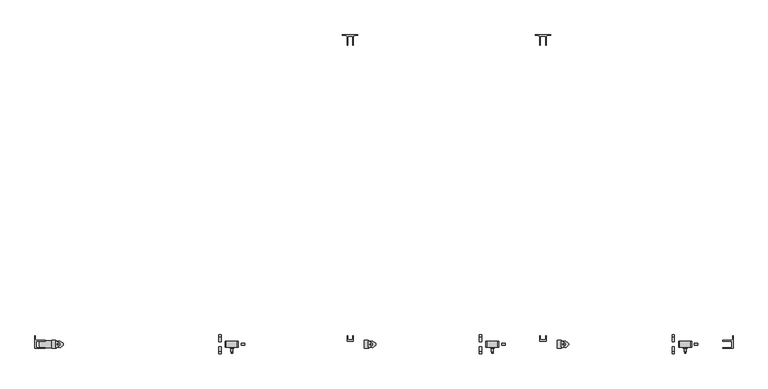
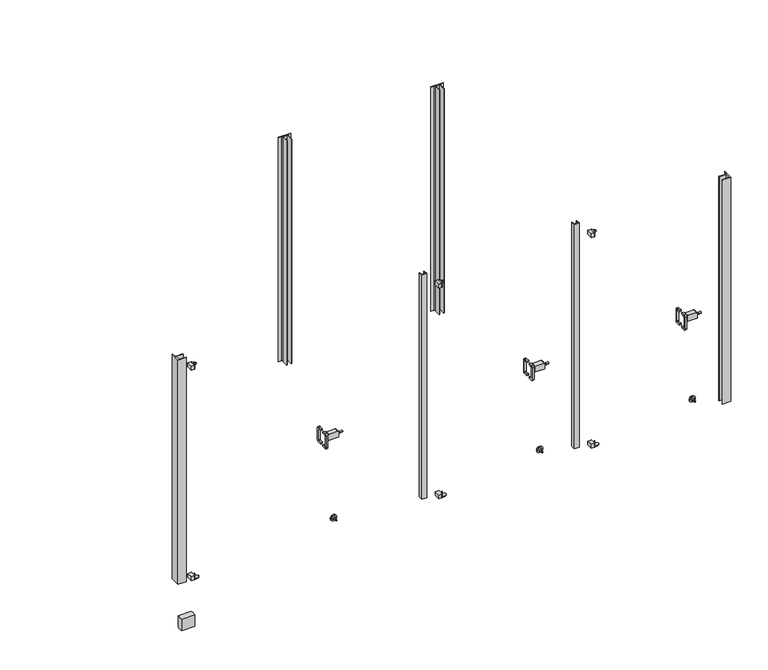
"""IFC4 building model written with IfcOpenShell, lengths in millimetres: proxy geometry, Partition-Floor_Braced-Bradley_Corp-St_Stl-ADA-N_Stalls : ADA (optional) + n Standard Stalls."""

from ifc_helpers import new_model, si_unit, point, frame, frame_2d, origin, origin_with_axes, place, context, project, spatial, polyline, circle_curve, ellipse_curve, trimmed, segment, composite_curve, outline, extrude, source, transform, mapped, element, save
from ifc_brep_helpers import plane_surface, cylinder_surface, revolved_surface, advanced_brep


def specialty_equipment_1cc22914(model_context):
    return source(origin(), model_context, "Body", "SolidModel", [
        extrude(outline(composite_curve([segment(trimmed(circle_curve(frame_2d((-1469.3891724, 977.9)), 10.16), [point((-1469.3891724, 988.06))], [point((-1459.2291724, 977.9))], False, "CARTESIAN"), True, "CONTINUOUS"), segment(polyline([(-1459.2291724, 977.9), (-1459.2291724, 901.7)]), True, "CONTINUOUS"), segment(trimmed(circle_curve(frame_2d((-1469.3891724, 901.7)), 10.16), [point((-1459.2291724, 901.7))], [point((-1469.3891724, 891.54))], False, "CARTESIAN"), True, "CONTINUOUS"), segment(polyline([(-1469.3891724, 891.54), (-1492.2491724, 891.54), (-1492.2491724, 901.7), (-1469.3891724, 901.7)]), True, "CONTINUOUS"), segment(trimmed(circle_curve(frame_2d((-1469.3891724, 904.24)), 2.54), [point((-1469.3891724, 901.7))], [point((-1466.8491724, 904.24))], True, "CARTESIAN"), True, "CONTINUOUS"), segment(polyline([(-1466.8491724, 904.24), (-1466.8491724, 975.36)]), True, "CONTINUOUS"), segment(trimmed(circle_curve(frame_2d((-1469.3891724, 975.36)), 2.54), [point((-1466.8491724, 975.36))], [point((-1469.3891724, 977.9))], True, "CARTESIAN"), True, "CONTINUOUS"), segment(polyline([(-1469.3891724, 977.9), (-1492.2491724, 977.9), (-1492.2491724, 988.06), (-1469.3891724, 988.06)]), True, "CONTINUOUS")], self_intersect=False)), frame((1086.5228738, 0.0, 0.0), z_axis=(1.0, 0.0, 0.0), x_axis=(0.0, 1.0, 0.0)), (0.0, 0.0, 1.0), 11.4113578),
        extrude(outline(composite_curve([segment(polyline([(-1540.51, 988.06), (-1517.65, 988.06), (-1517.65, 977.9), (-1540.51, 977.9)]), True, "CONTINUOUS"), segment(trimmed(circle_curve(frame_2d((-1540.51, 975.36)), 2.54), [point((-1540.51, 977.9))], [point((-1543.05, 975.36))], True, "CARTESIAN"), True, "CONTINUOUS"), segment(polyline([(-1543.05, 975.36), (-1543.05, 904.24)]), True, "CONTINUOUS"), segment(trimmed(circle_curve(frame_2d((-1540.51, 904.24)), 2.54), [point((-1543.05, 904.24))], [point((-1540.51, 901.7))], True, "CARTESIAN"), True, "CONTINUOUS"), segment(polyline([(-1540.51, 901.7), (-1517.65, 901.7), (-1517.65, 891.54), (-1540.51, 891.54)]), True, "CONTINUOUS"), segment(trimmed(circle_curve(frame_2d((-1540.51, 901.7)), 10.16), [point((-1540.51, 891.54))], [point((-1550.67, 901.7))], False, "CARTESIAN"), True, "CONTINUOUS"), segment(polyline([(-1550.67, 901.7), (-1550.67, 977.9)]), True, "CONTINUOUS"), segment(trimmed(circle_curve(frame_2d((-1540.51, 977.9)), 10.16), [point((-1550.67, 977.9))], [point((-1540.51, 988.06))], False, "CARTESIAN"), True, "CONTINUOUS")], self_intersect=False)), frame((1086.5228738, 0.0, 0.0), z_axis=(1.0, 0.0, 0.0), x_axis=(0.0, 1.0, 0.0)), (0.0, 0.0, 1.0), 11.4113578),
        extrude(outline(composite_curve([segment(trimmed(circle_curve(frame_2d((406.4, 1150.9250547)), 3.4532283), [point((402.9467717, 1150.9250547))], [point((409.8532283, 1150.9250547))], False, "CARTESIAN"), True, "CONTINUOUS"), segment(trimmed(circle_curve(frame_2d((406.4, 1150.9250547)), 3.4532283), [point((409.8532283, 1150.9250547))], [point((402.9467717, 1150.9250547))], False, "CARTESIAN"), True, "CONTINUOUS")], self_intersect=False)), frame((0.0, -1548.13, 0.0), z_axis=(0.0, 1.0, 0.0), x_axis=(0.0, 0.0, 1.0)), (0.0, 0.0, 1.0), 7.62),
        advanced_brep(
        [(1150.9250547, -1517.65, 406.4), (1131.8750547, -1517.65, 406.4), (1169.9750547, -1517.65, 406.4), (1156.0050547, -1540.51, 406.4), (1145.8450547, -1540.51, 406.4), (1150.9250547, -1540.51, 406.4), (1156.0050547, -1525.27, 406.4), (1145.8450547, -1525.27, 406.4), (1161.0850547, -1520.19, 406.4), (1140.7650547, -1520.19, 406.4), (1169.9750547, -1520.19, 406.4), (1131.8750547, -1520.19, 406.4)],
        [
            (0, 1),
            (1, 2, circle_curve(frame((1150.9250547, -1517.65, 406.4), z_axis=(0.0, 1.0, 0.0), x_axis=(-1.0, 0.0, 0.0)), 19.05)),
            (2, 0),
            (2, 1, circle_curve(frame((1150.9250547, -1517.65, 406.4), z_axis=(0.0, 1.0, 0.0), x_axis=(-1.0, 0.0, 0.0)), 19.05)),
            (3, 4, circle_curve(frame((1150.9250547, -1540.51, 406.4), z_axis=(0.0, -1.0, 0.0), x_axis=(-1.0, 0.0, 0.0)), 5.08)),
            (4, 5),
            (5, 3),
            (4, 3, circle_curve(frame((1150.9250547, -1540.51, 406.4), z_axis=(0.0, -1.0, 0.0), x_axis=(-1.0, 0.0, 0.0)), 5.08)),
            (6, 7, circle_curve(frame((1150.9250547, -1525.27, 406.4), z_axis=(0.0, -1.0, 0.0), x_axis=(-1.0, 0.0, 0.0)), 5.08)),
            (7, 4),
            (3, 6),
            (7, 6, circle_curve(frame((1150.9250547, -1525.27, 406.4), z_axis=(0.0, -1.0, 0.0), x_axis=(-1.0, 0.0, 0.0)), 5.08)),
            (8, 9, circle_curve(frame((1150.9250547, -1520.19, 406.4), z_axis=(0.0, -1.0, 0.0), x_axis=(-1.0, 0.0, 0.0)), 10.16)),
            (9, 7, circle_curve(frame((1145.8450547, -1520.19, 406.4), z_axis=(0.0, 0.0, 1.0), x_axis=(0.0, -1.0, 0.0)), 5.08)),
            (6, 8, circle_curve(frame((1156.0050547, -1520.19, 406.4), z_axis=(0.0, 0.0, 1.0), x_axis=(0.0, -1.0, 0.0)), 5.08)),
            (9, 8, circle_curve(frame((1150.9250547, -1520.19, 406.4), z_axis=(0.0, -1.0, 0.0), x_axis=(-1.0, 0.0, 0.0)), 10.16)),
            (10, 11, circle_curve(frame((1150.9250547, -1520.19, 406.4), z_axis=(0.0, -1.0, 0.0), x_axis=(-1.0, 0.0, 0.0)), 19.05)),
            (11, 9),
            (8, 10),
            (11, 10, circle_curve(frame((1150.9250547, -1520.19, 406.4), z_axis=(0.0, -1.0, 0.0), x_axis=(-1.0, 0.0, 0.0)), 19.05)),
            (1, 11),
            (10, 2),
        ],
        [
            plane_surface(frame((1150.9250547, -1517.65, 406.4), z_axis=(0.0, 1.0, 0.0), x_axis=(-1.0, 0.0, 0.0))),
            plane_surface(frame((1150.9250547, -1540.51, 406.4), z_axis=(0.0, -1.0, 0.0), x_axis=(-1.0, 0.0, 0.0))),
            cylinder_surface(frame((1150.9250547, -1561.6297247, 406.4), z_axis=(0.0, 1.0, 0.0), x_axis=(-1.0, 0.0, 0.0)), 5.08),
            revolved_surface(trimmed(ellipse_curve(frame((1145.8450547, -1520.19, 406.4), z_axis=(0.0, 0.0, -1.0), x_axis=(0.0, -1.0, 0.0)), 5.08, 5.08), [point((1145.8450547, -1525.27, 406.4))], [point((1140.7650547, -1520.19, 406.4))], True, "CARTESIAN"), (1150.9250547, -1561.6297247, 406.4), (0.0, 1.0, 0.0)),
            plane_surface(frame((1150.9250547, -1520.19, 406.4), z_axis=(0.0, -1.0, 0.0), x_axis=(-1.0, 0.0, 0.0))),
            cylinder_surface(frame((1150.9250547, -1561.6297247, 406.4), z_axis=(0.0, 1.0, 0.0), x_axis=(-1.0, 0.0, 0.0)), 19.05),
        ],
        [
            (0, [[1, 2, 3]]),
            (0, [[-3, 4, -1]]),
            (1, [[5, 6, 7]]),
            (1, [[8, -7, -6]]),
            (2, [[9, 10, -5, 11]]),
            (2, [[12, -11, -8, -10]]),
            (3, [[13, 14, -9, 15]]),
            (3, [[16, -15, -12, -14]]),
            (4, [[17, 18, -13, 19]]),
            (4, [[20, -19, -16, -18]]),
            (5, [[-2, 21, -17, 22]]),
            (5, [[-4, -22, -20, -21]]),
        ],
    ),
        advanced_brep(
        [(1195.3750547, -1499.87, 939.8), (1195.3750547, -1510.03, 939.8), (1212.8502547, -1510.03, 939.8), (1212.8502547, -1499.87, 939.8), (1195.3750547, -1504.95, 939.8), (1212.8502547, -1504.95, 939.8)],
        [
            (0, 1, circle_curve(frame((1195.3750547, -1504.95, 939.8), z_axis=(1.0, 0.0, 0.0), x_axis=(0.0, -1.0, 0.0)), 5.08)),
            (1, 2),
            (2, 3, circle_curve(frame((1212.8502547, -1504.95, 939.8), z_axis=(-1.0, 0.0, 0.0), x_axis=(0.0, -1.0, 0.0)), 5.08)),
            (3, 0),
            (1, 0, circle_curve(frame((1195.3750547, -1504.95, 939.8), z_axis=(1.0, 0.0, 0.0), x_axis=(0.0, -1.0, 0.0)), 5.08)),
            (3, 2, circle_curve(frame((1212.8502547, -1504.95, 939.8), z_axis=(-1.0, 0.0, 0.0), x_axis=(0.0, -1.0, 0.0)), 5.08)),
            (4, 1),
            (0, 4),
            (2, 5),
            (5, 3),
        ],
        [
            cylinder_surface(frame((1212.8502547, -1504.95, 939.8), z_axis=(-1.0, 0.0, 0.0), x_axis=(0.0, -1.0, 0.0)), 5.08),
            plane_surface(frame((1195.3750547, -1504.95, 939.8), z_axis=(-1.0, 0.0, 0.0), x_axis=(0.0, -1.0, 0.0))),
            plane_surface(frame((1212.8502547, -1504.95, 939.8), z_axis=(1.0, 0.0, 0.0), x_axis=(0.0, -1.0, 0.0))),
        ],
        [
            (0, [[1, 2, 3, 4]]),
            (0, [[5, -4, 6, -2]]),
            (1, [[7, -1, 8]]),
            (1, [[-8, -5, -7]]),
            (2, [[-3, 9, 10]]),
            (2, [[-6, -10, -9]]),
        ],
    ),
        extrude(outline(composite_curve([segment(trimmed(circle_curve(frame_2d((926.0058992, 1124.4309539)), 5.2558992), [point((926.0058992, 1119.1750547))], [point((920.75, 1124.4309539))], False, "CARTESIAN"), True, "CONTINUOUS"), segment(polyline([(920.75, 1124.4309539), (920.75, 1177.4191555)]), True, "CONTINUOUS"), segment(trimmed(circle_curve(frame_2d((926.0058992, 1177.4191555)), 5.2558992), [point((920.75, 1177.4191555))], [point((926.0058992, 1182.6750547))], False, "CARTESIAN"), True, "CONTINUOUS"), segment(polyline([(926.0058992, 1182.6750547), (953.5941008, 1182.6750547)]), True, "CONTINUOUS"), segment(trimmed(circle_curve(frame_2d((953.5941008, 1177.4191555)), 5.2558992), [point((953.5941008, 1182.6750547))], [point((958.85, 1177.4191555))], False, "CARTESIAN"), True, "CONTINUOUS"), segment(polyline([(958.85, 1177.4191555), (958.85, 1124.4309539)]), True, "CONTINUOUS"), segment(trimmed(circle_curve(frame_2d((953.5941008, 1124.4309539)), 5.2558992), [point((958.85, 1124.4309539))], [point((953.5941008, 1119.1750547))], False, "CARTESIAN"), True, "CONTINUOUS"), segment(polyline([(953.5941008, 1119.1750547), (926.0058992, 1119.1750547)]), True, "CONTINUOUS")], self_intersect=False)), frame((0.0, -1519.555, 0.0), z_axis=(0.0, 1.0, 0.0), x_axis=(0.0, 0.0, 1.0)), (0.0, 0.0, 1.0), 29.21),
        extrude(outline(composite_curve([segment(trimmed(circle_curve(frame_2d((-1469.3891724, 977.9)), 10.16), [point((-1469.3891724, 988.06))], [point((-1459.2291724, 977.9))], False, "CARTESIAN"), True, "CONTINUOUS"), segment(polyline([(-1459.2291724, 977.9), (-1459.2291724, 901.7)]), True, "CONTINUOUS"), segment(trimmed(circle_curve(frame_2d((-1469.3891724, 901.7)), 10.16), [point((-1459.2291724, 901.7))], [point((-1469.3891724, 891.54))], False, "CARTESIAN"), True, "CONTINUOUS"), segment(polyline([(-1469.3891724, 891.54), (-1492.2491724, 891.54), (-1492.2491724, 901.7), (-1469.3891724, 901.7)]), True, "CONTINUOUS"), segment(trimmed(circle_curve(frame_2d((-1469.3891724, 904.24)), 2.54), [point((-1469.3891724, 901.7))], [point((-1466.8491724, 904.24))], True, "CARTESIAN"), True, "CONTINUOUS"), segment(polyline([(-1466.8491724, 904.24), (-1466.8491724, 975.36)]), True, "CONTINUOUS"), segment(trimmed(circle_curve(frame_2d((-1469.3891724, 975.36)), 2.54), [point((-1466.8491724, 975.36))], [point((-1469.3891724, 977.9))], True, "CARTESIAN"), True, "CONTINUOUS"), segment(polyline([(-1469.3891724, 977.9), (-1492.2491724, 977.9), (-1492.2491724, 988.06), (-1469.3891724, 988.06)]), True, "CONTINUOUS")], self_intersect=False)), frame((2356.5228738, 0.0, 0.0), z_axis=(1.0, 0.0, 0.0), x_axis=(0.0, 1.0, 0.0)), (0.0, 0.0, 1.0), 11.4113578),
        extrude(outline(composite_curve([segment(polyline([(-1540.51, 988.06), (-1517.65, 988.06), (-1517.65, 977.9), (-1540.51, 977.9)]), True, "CONTINUOUS"), segment(trimmed(circle_curve(frame_2d((-1540.51, 975.36)), 2.54), [point((-1540.51, 977.9))], [point((-1543.05, 975.36))], True, "CARTESIAN"), True, "CONTINUOUS"), segment(polyline([(-1543.05, 975.36), (-1543.05, 904.24)]), True, "CONTINUOUS"), segment(trimmed(circle_curve(frame_2d((-1540.51, 904.24)), 2.54), [point((-1543.05, 904.24))], [point((-1540.51, 901.7))], True, "CARTESIAN"), True, "CONTINUOUS"), segment(polyline([(-1540.51, 901.7), (-1517.65, 901.7), (-1517.65, 891.54), (-1540.51, 891.54)]), True, "CONTINUOUS"), segment(trimmed(circle_curve(frame_2d((-1540.51, 901.7)), 10.16), [point((-1540.51, 891.54))], [point((-1550.67, 901.7))], False, "CARTESIAN"), True, "CONTINUOUS"), segment(polyline([(-1550.67, 901.7), (-1550.67, 977.9)]), True, "CONTINUOUS"), segment(trimmed(circle_curve(frame_2d((-1540.51, 977.9)), 10.16), [point((-1550.67, 977.9))], [point((-1540.51, 988.06))], False, "CARTESIAN"), True, "CONTINUOUS")], self_intersect=False)), frame((2356.5228738, 0.0, 0.0), z_axis=(1.0, 0.0, 0.0), x_axis=(0.0, 1.0, 0.0)), (0.0, 0.0, 1.0), 11.4113578),
        extrude(outline(composite_curve([segment(trimmed(circle_curve(frame_2d((406.4, 2420.9250547)), 3.4532283), [point((402.9467717, 2420.9250547))], [point((409.8532283, 2420.9250547))], False, "CARTESIAN"), True, "CONTINUOUS"), segment(trimmed(circle_curve(frame_2d((406.4, 2420.9250547)), 3.4532283), [point((409.8532283, 2420.9250547))], [point((402.9467717, 2420.9250547))], False, "CARTESIAN"), True, "CONTINUOUS")], self_intersect=False)), frame((0.0, -1548.13, 0.0), z_axis=(0.0, 1.0, 0.0), x_axis=(0.0, 0.0, 1.0)), (0.0, 0.0, 1.0), 7.62),
        advanced_brep(
        [(2420.9250547, -1517.65, 406.4), (2401.8750547, -1517.65, 406.4), (2439.9750547, -1517.65, 406.4), (2426.0050547, -1540.51, 406.4), (2415.8450547, -1540.51, 406.4), (2420.9250547, -1540.51, 406.4), (2426.0050547, -1525.27, 406.4), (2415.8450547, -1525.27, 406.4), (2431.0850547, -1520.19, 406.4), (2410.7650547, -1520.19, 406.4), (2439.9750547, -1520.19, 406.4), (2401.8750547, -1520.19, 406.4)],
        [
            (0, 1),
            (1, 2, circle_curve(frame((2420.9250547, -1517.65, 406.4), z_axis=(0.0, 1.0, 0.0), x_axis=(-1.0, 0.0, 0.0)), 19.05)),
            (2, 0),
            (2, 1, circle_curve(frame((2420.9250547, -1517.65, 406.4), z_axis=(0.0, 1.0, 0.0), x_axis=(-1.0, 0.0, 0.0)), 19.05)),
            (3, 4, circle_curve(frame((2420.9250547, -1540.51, 406.4), z_axis=(0.0, -1.0, 0.0), x_axis=(-1.0, 0.0, 0.0)), 5.08)),
            (4, 5),
            (5, 3),
            (4, 3, circle_curve(frame((2420.9250547, -1540.51, 406.4), z_axis=(0.0, -1.0, 0.0), x_axis=(-1.0, 0.0, 0.0)), 5.08)),
            (6, 7, circle_curve(frame((2420.9250547, -1525.27, 406.4), z_axis=(0.0, -1.0, 0.0), x_axis=(-1.0, 0.0, 0.0)), 5.08)),
            (7, 4),
            (3, 6),
            (7, 6, circle_curve(frame((2420.9250547, -1525.27, 406.4), z_axis=(0.0, -1.0, 0.0), x_axis=(-1.0, 0.0, 0.0)), 5.08)),
            (8, 9, circle_curve(frame((2420.9250547, -1520.19, 406.4), z_axis=(0.0, -1.0, 0.0), x_axis=(-1.0, 0.0, 0.0)), 10.16)),
            (9, 7, circle_curve(frame((2415.8450547, -1520.19, 406.4), z_axis=(0.0, 0.0, 1.0), x_axis=(0.0, -1.0, 0.0)), 5.08)),
            (6, 8, circle_curve(frame((2426.0050547, -1520.19, 406.4), z_axis=(0.0, 0.0, 1.0), x_axis=(0.0, -1.0, 0.0)), 5.08)),
            (9, 8, circle_curve(frame((2420.9250547, -1520.19, 406.4), z_axis=(0.0, -1.0, 0.0), x_axis=(-1.0, 0.0, 0.0)), 10.16)),
            (10, 11, circle_curve(frame((2420.9250547, -1520.19, 406.4), z_axis=(0.0, -1.0, 0.0), x_axis=(-1.0, 0.0, 0.0)), 19.05)),
            (11, 9),
            (8, 10),
            (11, 10, circle_curve(frame((2420.9250547, -1520.19, 406.4), z_axis=(0.0, -1.0, 0.0), x_axis=(-1.0, 0.0, 0.0)), 19.05)),
            (1, 11),
            (10, 2),
        ],
        [
            plane_surface(frame((2420.9250547, -1517.65, 406.4), z_axis=(0.0, 1.0, 0.0), x_axis=(-1.0, 0.0, 0.0))),
            plane_surface(frame((2420.9250547, -1540.51, 406.4), z_axis=(0.0, -1.0, 0.0), x_axis=(-1.0, 0.0, 0.0))),
            cylinder_surface(frame((2420.9250547, -1561.6297247, 406.4), z_axis=(0.0, 1.0, 0.0), x_axis=(-1.0, 0.0, 0.0)), 5.08),
            revolved_surface(trimmed(ellipse_curve(frame((2415.8450547, -1520.19, 406.4), z_axis=(0.0, 0.0, -1.0), x_axis=(0.0, -1.0, 0.0)), 5.08, 5.08), [point((2415.8450547, -1525.27, 406.4))], [point((2410.7650547, -1520.19, 406.4))], True, "CARTESIAN"), (2420.9250547, -1561.6297247, 406.4), (0.0, 1.0, 0.0)),
            plane_surface(frame((2420.9250547, -1520.19, 406.4), z_axis=(0.0, -1.0, 0.0), x_axis=(-1.0, 0.0, 0.0))),
            cylinder_surface(frame((2420.9250547, -1561.6297247, 406.4), z_axis=(0.0, 1.0, 0.0), x_axis=(-1.0, 0.0, 0.0)), 19.05),
        ],
        [
            (0, [[1, 2, 3]]),
            (0, [[-3, 4, -1]]),
            (1, [[5, 6, 7]]),
            (1, [[8, -7, -6]]),
            (2, [[9, 10, -5, 11]]),
            (2, [[12, -11, -8, -10]]),
            (3, [[13, 14, -9, 15]]),
            (3, [[16, -15, -12, -14]]),
            (4, [[17, 18, -13, 19]]),
            (4, [[20, -19, -16, -18]]),
            (5, [[-2, 21, -17, 22]]),
            (5, [[-4, -22, -20, -21]]),
        ],
    ),
        advanced_brep(
        [(2465.3750547, -1499.87, 939.8), (2465.3750547, -1510.03, 939.8), (2482.8502547, -1510.03, 939.8), (2482.8502547, -1499.87, 939.8), (2465.3750547, -1504.95, 939.8), (2482.8502547, -1504.95, 939.8)],
        [
            (0, 1, circle_curve(frame((2465.3750547, -1504.95, 939.8), z_axis=(1.0, 0.0, 0.0), x_axis=(0.0, -1.0, 0.0)), 5.08)),
            (1, 2),
            (2, 3, circle_curve(frame((2482.8502547, -1504.95, 939.8), z_axis=(-1.0, 0.0, 0.0), x_axis=(0.0, -1.0, 0.0)), 5.08)),
            (3, 0),
            (1, 0, circle_curve(frame((2465.3750547, -1504.95, 939.8), z_axis=(1.0, 0.0, 0.0), x_axis=(0.0, -1.0, 0.0)), 5.08)),
            (3, 2, circle_curve(frame((2482.8502547, -1504.95, 939.8), z_axis=(-1.0, 0.0, 0.0), x_axis=(0.0, -1.0, 0.0)), 5.08)),
            (4, 1),
            (0, 4),
            (2, 5),
            (5, 3),
        ],
        [
            cylinder_surface(frame((2482.8502547, -1504.95, 939.8), z_axis=(-1.0, 0.0, 0.0), x_axis=(0.0, -1.0, 0.0)), 5.08),
            plane_surface(frame((2465.3750547, -1504.95, 939.8), z_axis=(-1.0, 0.0, 0.0), x_axis=(0.0, -1.0, 0.0))),
            plane_surface(frame((2482.8502547, -1504.95, 939.8), z_axis=(1.0, 0.0, 0.0), x_axis=(0.0, -1.0, 0.0))),
        ],
        [
            (0, [[1, 2, 3, 4]]),
            (0, [[5, -4, 6, -2]]),
            (1, [[7, -1, 8]]),
            (1, [[-8, -5, -7]]),
            (2, [[-3, 9, 10]]),
            (2, [[-6, -10, -9]]),
        ],
    ),
        extrude(outline(composite_curve([segment(trimmed(circle_curve(frame_2d((926.0058992, 2394.4309539)), 5.2558992), [point((926.0058992, 2389.1750547))], [point((920.75, 2394.4309539))], False, "CARTESIAN"), True, "CONTINUOUS"), segment(polyline([(920.75, 2394.4309539), (920.75, 2447.4191555)]), True, "CONTINUOUS"), segment(trimmed(circle_curve(frame_2d((926.0058992, 2447.4191555)), 5.2558992), [point((920.75, 2447.4191555))], [point((926.0058992, 2452.6750547))], False, "CARTESIAN"), True, "CONTINUOUS"), segment(polyline([(926.0058992, 2452.6750547), (953.5941008, 2452.6750547)]), True, "CONTINUOUS"), segment(trimmed(circle_curve(frame_2d((953.5941008, 2447.4191555)), 5.2558992), [point((953.5941008, 2452.6750547))], [point((958.85, 2447.4191555))], False, "CARTESIAN"), True, "CONTINUOUS"), segment(polyline([(958.85, 2447.4191555), (958.85, 2394.4309539)]), True, "CONTINUOUS"), segment(trimmed(circle_curve(frame_2d((953.5941008, 2394.4309539)), 5.2558992), [point((958.85, 2394.4309539))], [point((953.5941008, 2389.1750547))], False, "CARTESIAN"), True, "CONTINUOUS"), segment(polyline([(953.5941008, 2389.1750547), (926.0058992, 2389.1750547)]), True, "CONTINUOUS")], self_intersect=False)), frame((0.0, -1519.555, 0.0), z_axis=(0.0, 1.0, 0.0), x_axis=(0.0, 0.0, 1.0)), (0.0, 0.0, 1.0), 29.21),
        extrude(outline(composite_curve([segment(trimmed(circle_curve(frame_2d((-1469.3891724, 977.9)), 10.16), [point((-1469.3891724, 988.06))], [point((-1459.2291724, 977.9))], False, "CARTESIAN"), True, "CONTINUOUS"), segment(polyline([(-1459.2291724, 977.9), (-1459.2291724, 901.7)]), True, "CONTINUOUS"), segment(trimmed(circle_curve(frame_2d((-1469.3891724, 901.7)), 10.16), [point((-1459.2291724, 901.7))], [point((-1469.3891724, 891.54))], False, "CARTESIAN"), True, "CONTINUOUS"), segment(polyline([(-1469.3891724, 891.54), (-1492.2491724, 891.54), (-1492.2491724, 901.7), (-1469.3891724, 901.7)]), True, "CONTINUOUS"), segment(trimmed(circle_curve(frame_2d((-1469.3891724, 904.24)), 2.54), [point((-1469.3891724, 901.7))], [point((-1466.8491724, 904.24))], True, "CARTESIAN"), True, "CONTINUOUS"), segment(polyline([(-1466.8491724, 904.24), (-1466.8491724, 975.36)]), True, "CONTINUOUS"), segment(trimmed(circle_curve(frame_2d((-1469.3891724, 975.36)), 2.54), [point((-1466.8491724, 975.36))], [point((-1469.3891724, 977.9))], True, "CARTESIAN"), True, "CONTINUOUS"), segment(polyline([(-1469.3891724, 977.9), (-1492.2491724, 977.9), (-1492.2491724, 988.06), (-1469.3891724, 988.06)]), True, "CONTINUOUS")], self_intersect=False)), frame((3296.3228738, 0.0, 0.0), z_axis=(1.0, 0.0, 0.0), x_axis=(0.0, 1.0, 0.0)), (0.0, 0.0, 1.0), 11.4113578),
        extrude(outline(composite_curve([segment(polyline([(-1540.51, 988.06), (-1517.65, 988.06), (-1517.65, 977.9), (-1540.51, 977.9)]), True, "CONTINUOUS"), segment(trimmed(circle_curve(frame_2d((-1540.51, 975.36)), 2.54), [point((-1540.51, 977.9))], [point((-1543.05, 975.36))], True, "CARTESIAN"), True, "CONTINUOUS"), segment(polyline([(-1543.05, 975.36), (-1543.05, 904.24)]), True, "CONTINUOUS"), segment(trimmed(circle_curve(frame_2d((-1540.51, 904.24)), 2.54), [point((-1543.05, 904.24))], [point((-1540.51, 901.7))], True, "CARTESIAN"), True, "CONTINUOUS"), segment(polyline([(-1540.51, 901.7), (-1517.65, 901.7), (-1517.65, 891.54), (-1540.51, 891.54)]), True, "CONTINUOUS"), segment(trimmed(circle_curve(frame_2d((-1540.51, 901.7)), 10.16), [point((-1540.51, 891.54))], [point((-1550.67, 901.7))], False, "CARTESIAN"), True, "CONTINUOUS"), segment(polyline([(-1550.67, 901.7), (-1550.67, 977.9)]), True, "CONTINUOUS"), segment(trimmed(circle_curve(frame_2d((-1540.51, 977.9)), 10.16), [point((-1550.67, 977.9))], [point((-1540.51, 988.06))], False, "CARTESIAN"), True, "CONTINUOUS")], self_intersect=False)), frame((3296.3228738, 0.0, 0.0), z_axis=(1.0, 0.0, 0.0), x_axis=(0.0, 1.0, 0.0)), (0.0, 0.0, 1.0), 11.4113578),
        extrude(outline(composite_curve([segment(trimmed(circle_curve(frame_2d((406.4, 3360.7250547)), 3.4532283), [point((402.9467717, 3360.7250547))], [point((409.8532283, 3360.7250547))], False, "CARTESIAN"), True, "CONTINUOUS"), segment(trimmed(circle_curve(frame_2d((406.4, 3360.7250547)), 3.4532283), [point((409.8532283, 3360.7250547))], [point((402.9467717, 3360.7250547))], False, "CARTESIAN"), True, "CONTINUOUS")], self_intersect=False)), frame((0.0, -1548.13, 0.0), z_axis=(0.0, 1.0, 0.0), x_axis=(0.0, 0.0, 1.0)), (0.0, 0.0, 1.0), 7.62),
        advanced_brep(
        [(3360.7250547, -1517.65, 406.4), (3341.6750547, -1517.65, 406.4), (3379.7750547, -1517.65, 406.4), (3365.8050547, -1540.51, 406.4), (3355.6450547, -1540.51, 406.4), (3360.7250547, -1540.51, 406.4), (3365.8050547, -1525.27, 406.4), (3355.6450547, -1525.27, 406.4), (3370.8850547, -1520.19, 406.4), (3350.5650547, -1520.19, 406.4), (3379.7750547, -1520.19, 406.4), (3341.6750547, -1520.19, 406.4)],
        [
            (0, 1),
            (1, 2, circle_curve(frame((3360.7250547, -1517.65, 406.4), z_axis=(0.0, 1.0, 0.0), x_axis=(-1.0, 0.0, 0.0)), 19.05)),
            (2, 0),
            (2, 1, circle_curve(frame((3360.7250547, -1517.65, 406.4), z_axis=(0.0, 1.0, 0.0), x_axis=(-1.0, 0.0, 0.0)), 19.05)),
            (3, 4, circle_curve(frame((3360.7250547, -1540.51, 406.4), z_axis=(0.0, -1.0, 0.0), x_axis=(-1.0, 0.0, 0.0)), 5.08)),
            (4, 5),
            (5, 3),
            (4, 3, circle_curve(frame((3360.7250547, -1540.51, 406.4), z_axis=(0.0, -1.0, 0.0), x_axis=(-1.0, 0.0, 0.0)), 5.08)),
            (6, 7, circle_curve(frame((3360.7250547, -1525.27, 406.4), z_axis=(0.0, -1.0, 0.0), x_axis=(-1.0, 0.0, 0.0)), 5.08)),
            (7, 4),
            (3, 6),
            (7, 6, circle_curve(frame((3360.7250547, -1525.27, 406.4), z_axis=(0.0, -1.0, 0.0), x_axis=(-1.0, 0.0, 0.0)), 5.08)),
            (8, 9, circle_curve(frame((3360.7250547, -1520.19, 406.4), z_axis=(0.0, -1.0, 0.0), x_axis=(-1.0, 0.0, 0.0)), 10.16)),
            (9, 7, circle_curve(frame((3355.6450547, -1520.19, 406.4), z_axis=(0.0, 0.0, 1.0), x_axis=(0.0, -1.0, 0.0)), 5.08)),
            (6, 8, circle_curve(frame((3365.8050547, -1520.19, 406.4), z_axis=(0.0, 0.0, 1.0), x_axis=(0.0, -1.0, 0.0)), 5.08)),
            (9, 8, circle_curve(frame((3360.7250547, -1520.19, 406.4), z_axis=(0.0, -1.0, 0.0), x_axis=(-1.0, 0.0, 0.0)), 10.16)),
            (10, 11, circle_curve(frame((3360.7250547, -1520.19, 406.4), z_axis=(0.0, -1.0, 0.0), x_axis=(-1.0, 0.0, 0.0)), 19.05)),
            (11, 9),
            (8, 10),
            (11, 10, circle_curve(frame((3360.7250547, -1520.19, 406.4), z_axis=(0.0, -1.0, 0.0), x_axis=(-1.0, 0.0, 0.0)), 19.05)),
            (1, 11),
            (10, 2),
        ],
        [
            plane_surface(frame((3360.7250547, -1517.65, 406.4), z_axis=(0.0, 1.0, 0.0), x_axis=(-1.0, 0.0, 0.0))),
            plane_surface(frame((3360.7250547, -1540.51, 406.4), z_axis=(0.0, -1.0, 0.0), x_axis=(-1.0, 0.0, 0.0))),
            cylinder_surface(frame((3360.7250547, -1561.6297247, 406.4), z_axis=(0.0, 1.0, 0.0), x_axis=(-1.0, 0.0, 0.0)), 5.08),
            revolved_surface(trimmed(ellipse_curve(frame((3355.6450547, -1520.19, 406.4), z_axis=(0.0, 0.0, -1.0), x_axis=(0.0, -1.0, 0.0)), 5.08, 5.08), [point((3355.6450547, -1525.27, 406.4))], [point((3350.5650547, -1520.19, 406.4))], True, "CARTESIAN"), (3360.7250547, -1561.6297247, 406.4), (0.0, 1.0, 0.0)),
            plane_surface(frame((3360.7250547, -1520.19, 406.4), z_axis=(0.0, -1.0, 0.0), x_axis=(-1.0, 0.0, 0.0))),
            cylinder_surface(frame((3360.7250547, -1561.6297247, 406.4), z_axis=(0.0, 1.0, 0.0), x_axis=(-1.0, 0.0, 0.0)), 19.05),
        ],
        [
            (0, [[1, 2, 3]]),
            (0, [[-3, 4, -1]]),
            (1, [[5, 6, 7]]),
            (1, [[8, -7, -6]]),
            (2, [[9, 10, -5, 11]]),
            (2, [[12, -11, -8, -10]]),
            (3, [[13, 14, -9, 15]]),
            (3, [[16, -15, -12, -14]]),
            (4, [[17, 18, -13, 19]]),
            (4, [[20, -19, -16, -18]]),
            (5, [[-2, 21, -17, 22]]),
            (5, [[-4, -22, -20, -21]]),
        ],
    ),
        advanced_brep(
        [(3405.1750547, -1499.87, 939.8), (3405.1750547, -1510.03, 939.8), (3422.6502547, -1510.03, 939.8), (3422.6502547, -1499.87, 939.8), (3405.1750547, -1504.95, 939.8), (3422.6502547, -1504.95, 939.8)],
        [
            (0, 1, circle_curve(frame((3405.1750547, -1504.95, 939.8), z_axis=(1.0, 0.0, 0.0), x_axis=(0.0, -1.0, 0.0)), 5.08)),
            (1, 2),
            (2, 3, circle_curve(frame((3422.6502547, -1504.95, 939.8), z_axis=(-1.0, 0.0, 0.0), x_axis=(0.0, -1.0, 0.0)), 5.08)),
            (3, 0),
            (1, 0, circle_curve(frame((3405.1750547, -1504.95, 939.8), z_axis=(1.0, 0.0, 0.0), x_axis=(0.0, -1.0, 0.0)), 5.08)),
            (3, 2, circle_curve(frame((3422.6502547, -1504.95, 939.8), z_axis=(-1.0, 0.0, 0.0), x_axis=(0.0, -1.0, 0.0)), 5.08)),
            (4, 1),
            (0, 4),
            (2, 5),
            (5, 3),
        ],
        [
            cylinder_surface(frame((3422.6502547, -1504.95, 939.8), z_axis=(-1.0, 0.0, 0.0), x_axis=(0.0, -1.0, 0.0)), 5.08),
            plane_surface(frame((3405.1750547, -1504.95, 939.8), z_axis=(-1.0, 0.0, 0.0), x_axis=(0.0, -1.0, 0.0))),
            plane_surface(frame((3422.6502547, -1504.95, 939.8), z_axis=(1.0, 0.0, 0.0), x_axis=(0.0, -1.0, 0.0))),
        ],
        [
            (0, [[1, 2, 3, 4]]),
            (0, [[5, -4, 6, -2]]),
            (1, [[7, -1, 8]]),
            (1, [[-8, -5, -7]]),
            (2, [[-3, 9, 10]]),
            (2, [[-6, -10, -9]]),
        ],
    ),
        extrude(outline(composite_curve([segment(trimmed(circle_curve(frame_2d((926.0058992, 3334.2309539)), 5.2558992), [point((926.0058992, 3328.9750547))], [point((920.75, 3334.2309539))], False, "CARTESIAN"), True, "CONTINUOUS"), segment(polyline([(920.75, 3334.2309539), (920.75, 3387.2191555)]), True, "CONTINUOUS"), segment(trimmed(circle_curve(frame_2d((926.0058992, 3387.2191555)), 5.2558992), [point((920.75, 3387.2191555))], [point((926.0058992, 3392.4750547))], False, "CARTESIAN"), True, "CONTINUOUS"), segment(polyline([(926.0058992, 3392.4750547), (953.5941008, 3392.4750547)]), True, "CONTINUOUS"), segment(trimmed(circle_curve(frame_2d((953.5941008, 3387.2191555)), 5.2558992), [point((953.5941008, 3392.4750547))], [point((958.85, 3387.2191555))], False, "CARTESIAN"), True, "CONTINUOUS"), segment(polyline([(958.85, 3387.2191555), (958.85, 3334.2309539)]), True, "CONTINUOUS"), segment(trimmed(circle_curve(frame_2d((953.5941008, 3334.2309539)), 5.2558992), [point((958.85, 3334.2309539))], [point((953.5941008, 3328.9750547))], False, "CARTESIAN"), True, "CONTINUOUS"), segment(polyline([(953.5941008, 3328.9750547), (926.0058992, 3328.9750547)]), True, "CONTINUOUS")], self_intersect=False)), frame((0.0, -1519.555, 0.0), z_axis=(0.0, 1.0, 0.0), x_axis=(0.0, 0.0, 1.0)), (0.0, 0.0, 1.0), 29.21),
        extrude(outline(composite_curve([segment(polyline([(3594.1002547, -1463.675), (3594.1002547, -1523.365), (3543.3002547, -1523.365), (3543.3002547, -1520.825), (3587.1524359, -1520.825), (3587.1524359, -1489.075), (3543.3002547, -1489.075), (3543.3002547, -1486.535), (3585.2102547, -1486.535)]), True, "CONTINUOUS"), segment(trimmed(circle_curve(frame_2d((3585.2102547, -1480.185)), 6.35), [point((3585.2102547, -1486.535))], [point((3591.5602547, -1480.185))], True, "CARTESIAN"), True, "CONTINUOUS"), segment(polyline([(3591.5602547, -1480.185), (3591.5602547, -1463.675), (3594.1002547, -1463.675)]), True, "CONTINUOUS")], self_intersect=False)), frame((0.0, 0.0, 311.15), z_axis=(0.0, 0.0, 1.0), x_axis=(1.0, 0.0, 0.0)), (0.0, 0.0, 1.0), 1460.5),
        extrude(outline(composite_curve([segment(trimmed(circle_curve(frame_2d((2765.7554547, -1504.95)), 2.54), [point((2765.7554547, -1507.49))], [point((2765.7554547, -1502.41))], False, "CARTESIAN"), True, "CONTINUOUS"), segment(trimmed(circle_curve(frame_2d((2765.7554547, -1504.95)), 2.54), [point((2765.7554547, -1502.41))], [point((2765.7554547, -1507.49))], False, "CARTESIAN"), True, "CONTINUOUS")], self_intersect=False)), frame((0.0, 0.0, 304.8), z_axis=(0.0, 0.0, 1.0), x_axis=(1.0, 0.0, 0.0)), (0.0, 0.0, 1.0), 25.4),
        extrude(outline(composite_curve([segment(polyline([(2755.9002547, -1489.71), (2777.4902547, -1489.075), (2787.6502547, -1497.33)]), True, "CONTINUOUS"), segment(trimmed(circle_curve(frame_2d((2783.8402547, -1504.95)), 8.519419), [point((2787.6502547, -1497.33))], [point((2787.6502547, -1512.57))], False, "CARTESIAN"), True, "CONTINUOUS"), segment(polyline([(2787.6502547, -1512.57), (2777.4902547, -1520.825), (2755.9002547, -1520.19), (2755.9002547, -1489.71)]), True, "CONTINUOUS")], self_intersect=False)), frame((0.0, 0.0, 304.8), z_axis=(0.0, 0.0, 1.0), x_axis=(1.0, 0.0, 0.0)), (0.0, 0.0, 1.0), 3.81),
        extrude(outline(composite_curve([segment(polyline([(2736.8502547, -1486.535), (2755.9002547, -1486.535)]), True, "CONTINUOUS"), segment(trimmed(circle_curve(frame_2d((2755.9002547, -1489.075)), 2.54), [point((2755.9002547, -1486.535))], [point((2758.4402547, -1489.075))], False, "CARTESIAN"), True, "CONTINUOUS"), segment(trimmed(circle_curve(frame_2d((2650.6397496, -1504.95)), 108.9631338), [point((2758.4402547, -1489.075))], [point((2758.4402547, -1520.825))], False, "CARTESIAN"), True, "CONTINUOUS"), segment(trimmed(circle_curve(frame_2d((2755.9002547, -1520.825)), 2.54), [point((2758.4402547, -1520.825))], [point((2755.9002547, -1523.365))], False, "CARTESIAN"), True, "CONTINUOUS"), segment(polyline([(2755.9002547, -1523.365), (2736.8502547, -1523.365), (2736.8502547, -1486.535)]), True, "CONTINUOUS")], self_intersect=False)), frame((0.0, 0.0, 304.8), z_axis=(0.0, 0.0, 1.0), x_axis=(1.0, 0.0, 0.0)), (0.0, 0.0, 1.0), 25.4),
        extrude(outline(composite_curve([segment(trimmed(circle_curve(frame_2d((2765.7554547, -1504.95)), 2.54), [point((2765.7554547, -1507.49))], [point((2765.7554547, -1502.41))], False, "CARTESIAN"), True, "CONTINUOUS"), segment(trimmed(circle_curve(frame_2d((2765.7554547, -1504.95)), 2.54), [point((2765.7554547, -1502.41))], [point((2765.7554547, -1507.49))], False, "CARTESIAN"), True, "CONTINUOUS")], self_intersect=False)), frame((0.0, 0.0, 1676.4), z_axis=(0.0, 0.0, 1.0), x_axis=(1.0, 0.0, 0.0)), (0.0, 0.0, 1.0), 25.4),
        extrude(outline(composite_curve([segment(polyline([(2760.6754547, -1520.825), (2755.9002547, -1520.19), (2755.9002547, -1489.71), (2760.6754547, -1489.075), (2770.8354547, -1497.33)]), True, "CONTINUOUS"), segment(trimmed(circle_curve(frame_2d((2767.0254547, -1504.95)), 8.519419), [point((2770.8354547, -1497.33))], [point((2770.8354547, -1512.57))], False, "CARTESIAN"), True, "CONTINUOUS"), segment(polyline([(2770.8354547, -1512.57), (2760.6754547, -1520.825)]), True, "CONTINUOUS")], self_intersect=False)), frame((0.0, 0.0, 1697.99), z_axis=(0.0, 0.0, 1.0), x_axis=(1.0, 0.0, 0.0)), (0.0, 0.0, 1.0), 3.81),
        extrude(outline(composite_curve([segment(polyline([(2736.8502547, -1486.535), (2755.9002547, -1486.535)]), True, "CONTINUOUS"), segment(trimmed(circle_curve(frame_2d((2755.9002547, -1489.075)), 2.54), [point((2755.9002547, -1486.535))], [point((2758.4402547, -1489.075))], False, "CARTESIAN"), True, "CONTINUOUS"), segment(trimmed(circle_curve(frame_2d((2650.6397496, -1504.95)), 108.9631338), [point((2758.4402547, -1489.075))], [point((2758.4402547, -1520.825))], False, "CARTESIAN"), True, "CONTINUOUS"), segment(trimmed(circle_curve(frame_2d((2755.9002547, -1520.825)), 2.54), [point((2758.4402547, -1520.825))], [point((2755.9002547, -1523.365))], False, "CARTESIAN"), True, "CONTINUOUS"), segment(polyline([(2755.9002547, -1523.365), (2736.8502547, -1523.365), (2736.8502547, -1486.535)]), True, "CONTINUOUS")], self_intersect=False)), frame((0.0, 0.0, 1676.4), z_axis=(0.0, 0.0, 1.0), x_axis=(1.0, 0.0, 0.0)), (0.0, 0.0, 1.0), 25.4),
        extrude(outline(composite_curve([segment(trimmed(circle_curve(frame_2d((1825.9554547, -1504.95)), 2.54), [point((1825.9554547, -1507.49))], [point((1825.9554547, -1502.41))], False, "CARTESIAN"), True, "CONTINUOUS"), segment(trimmed(circle_curve(frame_2d((1825.9554547, -1504.95)), 2.54), [point((1825.9554547, -1502.41))], [point((1825.9554547, -1507.49))], False, "CARTESIAN"), True, "CONTINUOUS")], self_intersect=False)), frame((0.0, 0.0, 304.8), z_axis=(0.0, 0.0, 1.0), x_axis=(1.0, 0.0, 0.0)), (0.0, 0.0, 1.0), 25.4),
        extrude(outline(composite_curve([segment(polyline([(1816.1002547, -1489.71), (1837.6902547, -1489.075), (1847.8502547, -1497.33)]), True, "CONTINUOUS"), segment(trimmed(circle_curve(frame_2d((1844.0402547, -1504.95)), 8.519419), [point((1847.8502547, -1497.33))], [point((1847.8502547, -1512.57))], False, "CARTESIAN"), True, "CONTINUOUS"), segment(polyline([(1847.8502547, -1512.57), (1837.6902547, -1520.825), (1816.1002547, -1520.19), (1816.1002547, -1489.71)]), True, "CONTINUOUS")], self_intersect=False)), frame((0.0, 0.0, 304.8), z_axis=(0.0, 0.0, 1.0), x_axis=(1.0, 0.0, 0.0)), (0.0, 0.0, 1.0), 3.81),
        extrude(outline(composite_curve([segment(polyline([(1797.0502547, -1486.535), (1816.1002547, -1486.535)]), True, "CONTINUOUS"), segment(trimmed(circle_curve(frame_2d((1816.1002547, -1489.075)), 2.54), [point((1816.1002547, -1486.535))], [point((1818.6402547, -1489.075))], False, "CARTESIAN"), True, "CONTINUOUS"), segment(trimmed(circle_curve(frame_2d((1710.8397496, -1504.95)), 108.9631338), [point((1818.6402547, -1489.075))], [point((1818.6402547, -1520.825))], False, "CARTESIAN"), True, "CONTINUOUS"), segment(trimmed(circle_curve(frame_2d((1816.1002547, -1520.825)), 2.54), [point((1818.6402547, -1520.825))], [point((1816.1002547, -1523.365))], False, "CARTESIAN"), True, "CONTINUOUS"), segment(polyline([(1816.1002547, -1523.365), (1797.0502547, -1523.365), (1797.0502547, -1486.535)]), True, "CONTINUOUS")], self_intersect=False)), frame((0.0, 0.0, 304.8), z_axis=(0.0, 0.0, 1.0), x_axis=(1.0, 0.0, 0.0)), (0.0, 0.0, 1.0), 25.4),
        extrude(outline(composite_curve([segment(trimmed(circle_curve(frame_2d((1825.9554547, -1504.95)), 2.54), [point((1825.9554547, -1507.49))], [point((1825.9554547, -1502.41))], False, "CARTESIAN"), True, "CONTINUOUS"), segment(trimmed(circle_curve(frame_2d((1825.9554547, -1504.95)), 2.54), [point((1825.9554547, -1502.41))], [point((1825.9554547, -1507.49))], False, "CARTESIAN"), True, "CONTINUOUS")], self_intersect=False)), frame((0.0, 0.0, 1676.4), z_axis=(0.0, 0.0, 1.0), x_axis=(1.0, 0.0, 0.0)), (0.0, 0.0, 1.0), 25.4),
        extrude(outline(composite_curve([segment(polyline([(1820.8754547, -1520.825), (1816.1002547, -1520.19), (1816.1002547, -1489.71), (1820.8754547, -1489.075), (1831.0354547, -1497.33)]), True, "CONTINUOUS"), segment(trimmed(circle_curve(frame_2d((1827.2254547, -1504.95)), 8.519419), [point((1831.0354547, -1497.33))], [point((1831.0354547, -1512.57))], False, "CARTESIAN"), True, "CONTINUOUS"), segment(polyline([(1831.0354547, -1512.57), (1820.8754547, -1520.825)]), True, "CONTINUOUS")], self_intersect=False)), frame((0.0, 0.0, 1697.99), z_axis=(0.0, 0.0, 1.0), x_axis=(1.0, 0.0, 0.0)), (0.0, 0.0, 1.0), 3.81),
        extrude(outline(composite_curve([segment(polyline([(1797.0502547, -1486.535), (1816.1002547, -1486.535)]), True, "CONTINUOUS"), segment(trimmed(circle_curve(frame_2d((1816.1002547, -1489.075)), 2.54), [point((1816.1002547, -1486.535))], [point((1818.6402547, -1489.075))], False, "CARTESIAN"), True, "CONTINUOUS"), segment(trimmed(circle_curve(frame_2d((1710.8397496, -1504.95)), 108.9631338), [point((1818.6402547, -1489.075))], [point((1818.6402547, -1520.825))], False, "CARTESIAN"), True, "CONTINUOUS"), segment(trimmed(circle_curve(frame_2d((1816.1002547, -1520.825)), 2.54), [point((1818.6402547, -1520.825))], [point((1816.1002547, -1523.365))], False, "CARTESIAN"), True, "CONTINUOUS"), segment(polyline([(1816.1002547, -1523.365), (1797.0502547, -1523.365), (1797.0502547, -1486.535)]), True, "CONTINUOUS")], self_intersect=False)), frame((0.0, 0.0, 1676.4), z_axis=(0.0, 0.0, 1.0), x_axis=(1.0, 0.0, 0.0)), (0.0, 0.0, 1.0), 25.4),
        extrude(outline(polyline([(2651.7602547, -1489.075), (2651.7602547, -1463.675), (2654.3002547, -1463.675), (2654.3002547, -1482.1271812), (2679.7002547, -1482.1271812), (2679.7002547, -1463.675), (2682.2402547, -1463.675), (2682.2402547, -1489.075), (2651.7602547, -1489.075)])), frame((0.0, 0.0, 311.15), z_axis=(0.0, 0.0, 1.0), x_axis=(1.0, 0.0, 0.0)), (0.0, 0.0, 1.0), 1460.5),
        extrude(outline(composite_curve([segment(polyline([(2705.1002547, 3.175), (2705.1002547, 0.635), (2688.5902547, 0.635)]), True, "CONTINUOUS"), segment(trimmed(circle_curve(frame_2d((2688.5902547, -5.715)), 6.35), [point((2688.5902547, 0.635))], [point((2682.2402547, -5.715))], True, "CARTESIAN"), True, "CONTINUOUS"), segment(polyline([(2682.2402547, -5.715), (2682.2402547, -47.625), (2679.7002547, -47.625), (2679.7002547, -3.7728188), (2654.3002547, -3.7728188), (2654.3002547, -47.625), (2651.7602547, -47.625), (2651.7602547, -5.715)]), True, "CONTINUOUS"), segment(trimmed(circle_curve(frame_2d((2645.4102547, -5.715)), 6.35), [point((2651.7602547, -5.715))], [point((2645.4102547, 0.635))], True, "CARTESIAN"), True, "CONTINUOUS"), segment(polyline([(2645.4102547, 0.635), (2628.9002547, 0.635), (2628.9002547, 3.175), (2705.1002547, 3.175)]), True, "CONTINUOUS")], self_intersect=False)), frame((0.0, 0.0, 311.15), z_axis=(0.0, 0.0, 1.0), x_axis=(1.0, 0.0, 0.0)), (0.0, 0.0, 1.0), 1460.5),
        extrude(outline(composite_curve([segment(trimmed(circle_curve(frame_2d((301.9554547, -1504.95)), 2.54), [point((301.9554547, -1507.49))], [point((301.9554547, -1502.41))], False, "CARTESIAN"), True, "CONTINUOUS"), segment(trimmed(circle_curve(frame_2d((301.9554547, -1504.95)), 2.54), [point((301.9554547, -1502.41))], [point((301.9554547, -1507.49))], False, "CARTESIAN"), True, "CONTINUOUS")], self_intersect=False)), frame((0.0, 0.0, 304.8), z_axis=(0.0, 0.0, 1.0), x_axis=(1.0, 0.0, 0.0)), (0.0, 0.0, 1.0), 25.4),
        extrude(outline(composite_curve([segment(polyline([(292.1002547, -1489.71), (313.6902547, -1489.075), (323.8502547, -1497.33)]), True, "CONTINUOUS"), segment(trimmed(circle_curve(frame_2d((320.0402547, -1504.95)), 8.519419), [point((323.8502547, -1497.33))], [point((323.8502547, -1512.57))], False, "CARTESIAN"), True, "CONTINUOUS"), segment(polyline([(323.8502547, -1512.57), (313.6902547, -1520.825), (292.1002547, -1520.19), (292.1002547, -1489.71)]), True, "CONTINUOUS")], self_intersect=False)), frame((0.0, 0.0, 304.8), z_axis=(0.0, 0.0, 1.0), x_axis=(1.0, 0.0, 0.0)), (0.0, 0.0, 1.0), 3.81),
        extrude(outline(composite_curve([segment(polyline([(273.0502547, -1486.535), (292.1002547, -1486.535)]), True, "CONTINUOUS"), segment(trimmed(circle_curve(frame_2d((292.1002547, -1489.075)), 2.54), [point((292.1002547, -1486.535))], [point((294.6402547, -1489.075))], False, "CARTESIAN"), True, "CONTINUOUS"), segment(trimmed(circle_curve(frame_2d((186.8397496, -1504.95)), 108.9631338), [point((294.6402547, -1489.075))], [point((294.6402547, -1520.825))], False, "CARTESIAN"), True, "CONTINUOUS"), segment(trimmed(circle_curve(frame_2d((292.1002547, -1520.825)), 2.54), [point((294.6402547, -1520.825))], [point((292.1002547, -1523.365))], False, "CARTESIAN"), True, "CONTINUOUS"), segment(polyline([(292.1002547, -1523.365), (273.0502547, -1523.365), (273.0502547, -1486.535)]), True, "CONTINUOUS")], self_intersect=False)), frame((0.0, 0.0, 304.8), z_axis=(0.0, 0.0, 1.0), x_axis=(1.0, 0.0, 0.0)), (0.0, 0.0, 1.0), 25.4),
        extrude(outline(composite_curve([segment(trimmed(circle_curve(frame_2d((301.9554547, -1504.95)), 2.54), [point((301.9554547, -1507.49))], [point((301.9554547, -1502.41))], False, "CARTESIAN"), True, "CONTINUOUS"), segment(trimmed(circle_curve(frame_2d((301.9554547, -1504.95)), 2.54), [point((301.9554547, -1502.41))], [point((301.9554547, -1507.49))], False, "CARTESIAN"), True, "CONTINUOUS")], self_intersect=False)), frame((0.0, 0.0, 1676.4), z_axis=(0.0, 0.0, 1.0), x_axis=(1.0, 0.0, 0.0)), (0.0, 0.0, 1.0), 25.4),
        extrude(outline(composite_curve([segment(polyline([(296.8754547, -1520.825), (292.1002547, -1520.19), (292.1002547, -1489.71), (296.8754547, -1489.075), (307.0354547, -1497.33)]), True, "CONTINUOUS"), segment(trimmed(circle_curve(frame_2d((303.2254547, -1504.95)), 8.519419), [point((307.0354547, -1497.33))], [point((307.0354547, -1512.57))], False, "CARTESIAN"), True, "CONTINUOUS"), segment(polyline([(307.0354547, -1512.57), (296.8754547, -1520.825)]), True, "CONTINUOUS")], self_intersect=False)), frame((0.0, 0.0, 1697.99), z_axis=(0.0, 0.0, 1.0), x_axis=(1.0, 0.0, 0.0)), (0.0, 0.0, 1.0), 3.81),
        extrude(outline(composite_curve([segment(polyline([(273.0502547, -1486.535), (292.1002547, -1486.535)]), True, "CONTINUOUS"), segment(trimmed(circle_curve(frame_2d((292.1002547, -1489.075)), 2.54), [point((292.1002547, -1486.535))], [point((294.6402547, -1489.075))], False, "CARTESIAN"), True, "CONTINUOUS"), segment(trimmed(circle_curve(frame_2d((186.8397496, -1504.95)), 108.9631338), [point((294.6402547, -1489.075))], [point((294.6402547, -1520.825))], False, "CARTESIAN"), True, "CONTINUOUS"), segment(trimmed(circle_curve(frame_2d((292.1002547, -1520.825)), 2.54), [point((294.6402547, -1520.825))], [point((292.1002547, -1523.365))], False, "CARTESIAN"), True, "CONTINUOUS"), segment(polyline([(292.1002547, -1523.365), (273.0502547, -1523.365), (273.0502547, -1486.535)]), True, "CONTINUOUS")], self_intersect=False)), frame((0.0, 0.0, 1676.4), z_axis=(0.0, 0.0, 1.0), x_axis=(1.0, 0.0, 0.0)), (0.0, 0.0, 1.0), 25.4),
        extrude(outline(composite_curve([segment(polyline([(190.5002547, -1463.675), (193.0402547, -1463.675), (193.0402547, -1480.185)]), True, "CONTINUOUS"), segment(trimmed(circle_curve(frame_2d((199.3902547, -1480.185)), 6.35), [point((193.0402547, -1480.185))], [point((199.3902547, -1486.535))], True, "CARTESIAN"), True, "CONTINUOUS"), segment(polyline([(199.3902547, -1486.535), (241.3002547, -1486.535), (241.3002547, -1489.075), (197.4480735, -1489.075), (197.4480735, -1520.825), (241.3002547, -1520.825), (241.3002547, -1523.365), (190.5002547, -1523.365), (190.5002547, -1463.675)]), True, "CONTINUOUS")], self_intersect=False)), frame((0.0, 0.0, 311.15), z_axis=(0.0, 0.0, 1.0), x_axis=(1.0, 0.0, 0.0)), (0.0, 0.0, 1.0), 1460.5),
        extrude(outline(polyline([(1711.9602547, -1489.075), (1711.9602547, -1463.675), (1714.5002547, -1463.675), (1714.5002547, -1482.1271812), (1739.9002547, -1482.1271812), (1739.9002547, -1463.675), (1742.4402547, -1463.675), (1742.4402547, -1489.075), (1711.9602547, -1489.075)])), frame((0.0, 0.0, 311.15), z_axis=(0.0, 0.0, 1.0), x_axis=(1.0, 0.0, 0.0)), (0.0, 0.0, 1.0), 1460.5),
        extrude(outline(composite_curve([segment(polyline([(1765.3002547, 3.175), (1765.3002547, 0.635), (1748.7902547, 0.635)]), True, "CONTINUOUS"), segment(trimmed(circle_curve(frame_2d((1748.7902547, -5.715)), 6.35), [point((1748.7902547, 0.635))], [point((1742.4402547, -5.715))], True, "CARTESIAN"), True, "CONTINUOUS"), segment(polyline([(1742.4402547, -5.715), (1742.4402547, -47.625), (1739.9002547, -47.625), (1739.9002547, -3.7728188), (1714.5002547, -3.7728188), (1714.5002547, -47.625), (1711.9602547, -47.625), (1711.9602547, -5.715)]), True, "CONTINUOUS"), segment(trimmed(circle_curve(frame_2d((1705.6102547, -5.715)), 6.35), [point((1711.9602547, -5.715))], [point((1705.6102547, 0.635))], True, "CARTESIAN"), True, "CONTINUOUS"), segment(polyline([(1705.6102547, 0.635), (1689.1002547, 0.635), (1689.1002547, 3.175), (1765.3002547, 3.175)]), True, "CONTINUOUS")], self_intersect=False)), frame((0.0, 0.0, 311.15), z_axis=(0.0, 0.0, 1.0), x_axis=(1.0, 0.0, 0.0)), (0.0, 0.0, 1.0), 1460.5),
        extrude(outline(composite_curve([segment(polyline([(214.3127547, -1487.4875), (293.6891337, -1487.4875)]), True, "CONTINUOUS"), segment(trimmed(circle_curve(frame_2d((237.900102, -1504.95)), 58.4581471), [point((293.6891337, -1487.4875))], [point((293.6891337, -1522.4125))], False, "CARTESIAN"), True, "CONTINUOUS"), segment(polyline([(293.6891337, -1522.4125), (214.3127547, -1522.4125)]), True, "CONTINUOUS"), segment(trimmed(circle_curve(frame_2d((270.1017864, -1504.95)), 58.4581471), [point((214.3127547, -1522.4125))], [point((214.3127547, -1487.4875))], False, "CARTESIAN"), True, "CONTINUOUS")], self_intersect=False)), origin_with_axes(), (0.0, 0.0, 1.0), 76.2),
    ])


if __name__ == "__main__":
    model = new_model("IFC4")
    model_context = context("Model", 3, world=origin())
    ifc_project = project(units=[si_unit("LENGTHUNIT", "METRE", prefix="MILLI")], contexts=[model_context])
    site = spatial("IfcSite", under=ifc_project)
    building = spatial("IfcBuilding", under=site)
    placement = place(None, origin())
    specialty_equipment_shape = specialty_equipment_1cc22914(model_context)
    element("IfcBuildingElementProxy", 1, Name="Partition-Floor_Braced-Bradley_Corp-St_Stl-ADA-N_Stalls : ADA (optional) + n Standard Stalls", ObjectType="Partition-Floor_Braced-Bradley_Corp-St_Stl-ADA-N_Stalls : ADA (optional) + n Standard Stalls", at=placement, inside=building, context=model_context, shape_type="MappedRepresentation", body=[
        mapped(specialty_equipment_shape, transform((0.0, 0.0, 0.0), x_axis=(1.0, 0.0, 0.0), y_axis=(0.0, 1.0, 0.0), z_axis=(0.0, 0.0, 1.0))),
    ])
    save(model, "model.ifc")

# Revit data of these elements
# Type "Partition-Floor_Braced-Bradley_Corp-St_Stl-ADA-N_Stalls : ADA (optional) + n Standard Stalls"
#   Keynote = "M10211313.01"
#   Warranty Information = "Warranted 15 years against rust out, 5 years on chrome hardware, lifetime of the partition on the stainless steel hardware."
#   Version = "1.3"
#   URL = "http://www.bradleycorp.com/"
#   Type Comments = "n/a"
#   Technical Data = "n/a"
#   Keynote = "M10211313.01"
#   OmniClass Title = "Toilet Compartment and Urinal Screens"
#   OmniClass Code = "23.15.11.15.11"
#   Modeling Code = "n/a"
#   Model = "Stainless Steel - Series 500 - Floor Braced"
#   Material Note = "Other Hardware Also Available - Please See www.bradleycorp.com"
#   Material = "Metal - Bradley Corp - Chrome"
#   MasterFormat Title = "Toilet Compartments"
#   MasterFormat Number = "10 21 13"
#   Manufacturer = "Bradley Corporation"
#   LEED Credit = ""
#   Industry Standards = "n/a"
#   Fire Rating = "n/a"
#   Description = "Restroom Partitions, Floor-Braced"
#   Copyright = "This Model Data is Property of Bradley Corporation"
#   Complies to NAFTA = "n/a"
#   Buy American Act = "To Be Determined"
#   Assembly Code = "C1010400"
#   ADA Compliant [instance default] = "Yes"
#   Width [instance default] = 11' - 5"
#   Top Hinge = 5' - 7"
#   Door Opening Standard [instance default] = 2' - 2"
#   Door Opening Angle [instance default] = 0.00°
#   MaskR [instance default] = 3' - 1"
#   Mask M [instance default] = 3' - 1"
#   Mask [instance default] = 5' - 1"
#   Shoe Height = 0' - 3"
#   RPn [instance default] = 0' - 1"
#   Pilaster Height = 5' - 10"
#   Latch to Edge = 0' - 2"
#   Latch Height = 3' - 1"
#   LPn [instance default] = 0' - 1"
#   Start STDA [instance default] = 0' - 0"
#   Start STD [instance default] = 5' - 5 1/2"
#   Start AMB [instance default] = 0' - 4 1/2"
#   Start STD2 [instance default] = 8' - 6 1/2"
#   Stall Width Standard [instance default] = 3' - 0"
#   Stall Depth [instance default] = 4' - 10 3/4"
#   Right Pilaster Width STD [instance default] = 0' - 3"
#   Pilaster Thickness = 0' - 1 1/4"
#   Percentage of Recycled Content = 0
#   Panel Thickness = 0' - 1"
#   Left Pilaster Width [instance default] = 0' - 4 1/2"
#   Height = 5' - 10"
#   Gap Side Wall Right [instance default] = 0' - 0"
#   Gap Side Wall Left [instance default] = 0' - 0"
#   Gap Pilaster Panel = 0' - 0 1/2"
#   Gap Back Wall [instance default] = 0' - 1"
#   End Right Pilaster = 0' - 0 1/2"
#   Door Width Standard [instance default] = 2' - 1.624"
#   Door Width ADA [instance default] = 2' - 11.624"
#   Door Thickness = 0' - 1"
#   Door Swing Angle [instance default] = 0.00°
#   Door Opening ADA [instance default] = 3' - 0"
#   Door Height = 4' - 10"
#   Door Handle Height = 3' - 1"
#   Door Gap = 0' - 0.188"
#   Depth [instance default] = 5' - 0"
#   CALC_Start STDs [instance default] = 5' - 5 1/2"
#   CALC_WidthA [instance default] = 3' - 1"
#   CALC_STDA Width [instance default] = 0' - 5"
#   CALC_STD2 Width [instance default] = 2' - 9"
#   CALC_RP [instance default] = 0' - 0"
#   CALC_Half Pilaster = 0' - 0 5/8"
#   CALC_Half Door Width = 0' - 11"
#   CALC_STD1 Width [instance default] = 2' - 9"
#   CALC_Left [instance default] = 0' - 4 1/2"
#   CALC_Half Panel = 0' - 0 1/2"
#   CALC_Angle [instance default] = 30.00°
#   CALC_AMB Width [instance default] = 4' - 9"
#   CALC_ADAngle [instance default] = 0.00°
#   CALC_ADADoorW [instance default] = 2' - 11.624"
#   CALC_ADADoorSwing [instance default] = 0.00°
#   CALC_ADADiff [instance default] = 2' - 0"
#   Bumper Height = 1' - 4"
#   Bottom Hinge = 1' - 0"
#   Bottom AFF = 1' - 0"
#   Brackets Top Height = 5' - 4"
#   Brackets Bottom Height = 1' - 6"
#   Right Pilaster Width AMB [instance default] = 0' - 3"
#   Stall Width ADA [instance default] = 5' - 0"
#   Outswing Door ADA [instance default] = yes
#   Instructions On-Off Visibility = yes
#   Outswing Door [instance default] = no
#   STDA [instance default] = no
#   STD2 [instance default] = yes
#   STD1 [instance default] = yes
#   RP STD2 [instance default] = yes
#   RP STD1 [instance default] = yes
#   RP AMB [instance default] = yes
#   Stalls Array [instance default] = 2
#   Right Panel [instance default] = yes
#   Stalls [instance default] = 3
#   Left Panel [instance default] = yes
#   Continuous Brackets [instance default] = yes
#   CALC_STD2Out [instance default] = no
#   CALC_STD1Out [instance default] = no
#   CALC_OutADA [instance default] = yes
#   CALC_NSTD2Out [instance default] = yes
#   CALC_NSTD1Out [instance default] = yes
#   CALC_NRP [instance default] = no
#   CALC_NOutADA [instance default] = no
#   CALC_NLF [instance default] = no
#   CALC_ADAOut [instance default] = yes
#   Brackets [instance default] = no
#   ADA Stall [instance default] = yes
#   Shoe Material = Metal - Bradley Corp - Stainless Steel Satin
#   Hardware Material = Metal - Bradley Corp - Chrome
#   Partition Material = Metal - Bradley Corp - Chrome
# Element 1 (IfcBuildingElementProxy, "Partition-Floor_Braced-Bradley_Corp-St_Stl-ADA-N_Stalls : ADA (optional) + n Standard Stalls")
#   Width = 11' - 2"
#   MaskR = 3' - 0 1/2"
#   Mask = 5' - 0 1/2"
#   RPn = 0' - 0"
#   LPn = 0' - 0"
#   Start STD = 5' - 4"
#   Start AMB = 0' - 4"
#   Start STD2 = 8' - 5"
#   Left Pilaster Width = 0' - 3"
#   Gap Side Wall Right = 0' - 1"
#   Gap Side Wall Left = 0' - 1"
#   CALC_Start STDs = 5' - 4"
#   CALC_STD2 Width = 2' - 6 1/2"
#   CALC_RP = -0' - 2 1/2"
#   CALC_Left = 0' - 4"
#   CALC_Angle = 0.00°
#   CALC_AMB Width = 4' - 8"
#   Outswing Door = yes
#   RP STD2 = no
#   Right Panel = no
#   Left Panel = no
#   CALC_STD2Out = yes
#   CALC_STD1Out = yes
#   CALC_NSTD2Out = no
#   CALC_NSTD1Out = no
#   CALC_NRP = yes
#   CALC_NLF = yes
#   Materials on its faces: "Metal - Bradley Corp - Chrome", "Metal - Bradley Corp - Stainless Steel Satin", "Plastic - Bradley Corp - Black"
# Materials
#   "Metal - Bradley Corp - Stainless Steel Satin": class "Metal", colour RGB 189 187 185, transparency 0
#   "Metal - Bradley Corp - Chrome": class "Metal", colour RGB 106 119 125, transparency 0, Cost = 0
#   "Plastic - Bradley Corp - Black": class "Plastic", colour RGB 5 5 5, transparency 0
